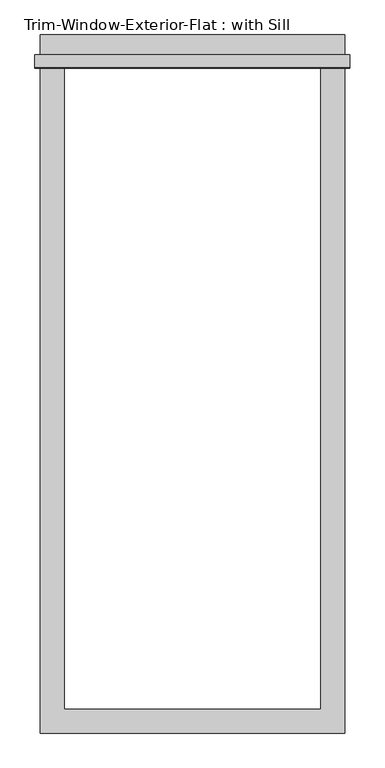
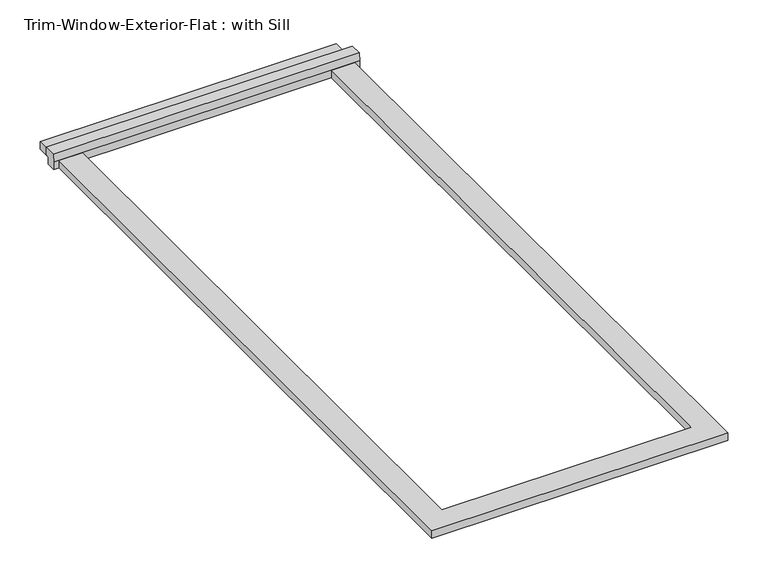
"""IFC4 building model written with IfcOpenShell, lengths in millimetres: proxy geometry, Trim-Window-Exterior-Flat : with Sill."""

from ifc_helpers import new_model, si_unit, frame, origin, origin_with_axes, place, context, project, spatial, polyline, outline, extrude, source, transform, mapped, element, save


def trim_window_exterior_flat_with_sill_419930c1(model_context):
    return source(origin(), model_context, "Body", "SweptSolid", [
        extrude(outline(polyline([(361.95, 1546.1823709), (-361.95, 1546.1823709), (-361.95, 1603.3323709), (361.95, 1603.3323709), (361.95, 1546.1823709)])), origin_with_axes(), (0.0, 0.0, 1.0), 19.05),
        extrude(outline(polyline([(1555.75, 38.1), (1555.75, 19.05), (1546.1823709, 19.05), (1546.1823709, 0.0), (1524.0, 0.0), (1524.0, 19.05), (1526.4580645, 38.1), (1555.75, 38.1)])), frame((-374.65, 0.0, 0.0), z_axis=(1.0, 0.0, 0.0), x_axis=(0.0, 1.0, 0.0)), (0.0, 0.0, 1.0), 749.3),
        extrude(outline(polyline([(-361.95, -57.15), (-361.95, 1524.0), (-304.8, 1524.0), (-304.8, 0.0), (304.8, 0.0), (304.8, 1524.0), (361.95, 1524.0), (361.95, -57.15), (-361.95, -57.15)])), origin_with_axes(), (0.0, 0.0, 1.0), 19.05),
    ])


if __name__ == "__main__":
    model = new_model("IFC4")
    model_context = context("Model", 3, world=origin())
    ifc_project = project(units=[si_unit("LENGTHUNIT", "METRE", prefix="MILLI")], contexts=[model_context])
    site = spatial("IfcSite", under=ifc_project)
    building = spatial("IfcBuilding", under=site)
    placement = place(None, origin())
    trim_window_exterior_flat_with_sill_shape = trim_window_exterior_flat_with_sill_419930c1(model_context)
    element("IfcBuildingElementProxy", 1, Name="Trim-Window-Exterior-Flat : with Sill", ObjectType="Trim-Window-Exterior-Flat : with Sill", at=placement, inside=building, context=model_context, shape_type="MappedRepresentation", body=[
        mapped(trim_window_exterior_flat_with_sill_shape, transform((0.0, 0.0, 0.0), x_axis=(1.0, 0.0, 0.0), y_axis=(0.0, 1.0, 0.0), z_axis=(0.0, 0.0, 1.0))),
    ])
    save(model, "model.ifc")

# Revit data of these elements
# Type "Trim-Window-Exterior-Flat : with Sill"
#   Trim Width = 0' - 2 1/4"
#   Trim Thickness_Picture Frame = 0' - 1 1/4"
#   Trim Thickness_with Sill = 0' - 0 3/4"
#   Sill Thickness = 0' - 1 1/4"
#   Opening Width [instance default] = 2' - 0"
#   Opening Height [instance default] = 3' - 0"
#   Default Elevation = 4' - 0"
#   Sill = yes
#   Picture Frame = no
#   Trim Material [instance default] = none
# Element 1 (IfcBuildingElementProxy, "Trim-Window-Exterior-Flat : with Sill")
#   Opening Height = 5' - 0"
#   Trim Material = Clad - White
#   Materials on its faces: "Clad - White"
# Materials
#   "Clad - White": class "Wood", colour RGB 242 242 238, transparency 0, Cost = 0
